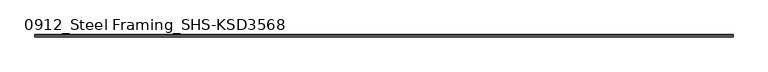
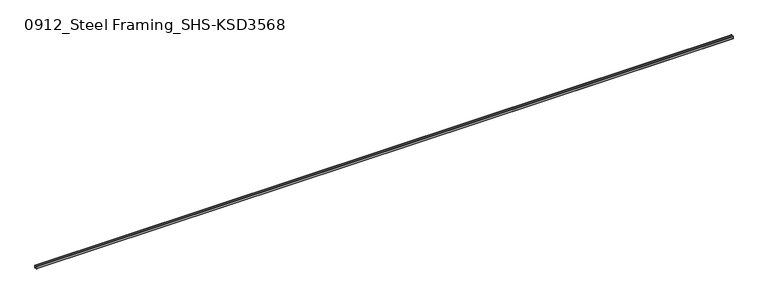
"""IFC4 building model written with IfcOpenShell, lengths in millimetres: beam geometry, 0912_Steel Framing_SHS-KSD3568 : H_SB_ASB_SHS-150x150x6."""

import ifcopenshell
import ifcopenshell.guid

model = None  # the IFC model being written
_history = None  # IfcOwnerHistory: only IFC2X3 demands one
_inside = {}  # id of a spatial element -> (the spatial element, [elements in it])
_under = {}  # id of a project, library or spatial element -> (it, [spatial elements below it])
_declared = {}  # id of a project -> (the project, [libraries it declares])
_typed = {}  # id of a type object -> (the type object, [elements of that type])
_made_of = {}  # id of a material, layer set ... -> (it, [elements and type objects made of it])


def new_model(schema):
    """Start an empty IFC model of exactly this schema.

    Asked for "IFC4X3", IfcOpenShell would pick the latest addendum, in which some entities
    have other attributes; the version numbers below select the first issue.
    IFC2X3 requires an IfcOwnerHistory on every rooted entity: one is made here for all.
    """
    global model, _history
    if schema == "IFC4X3":
        model = ifcopenshell.file(schema_version=(4, 3, 0, 0))
    else:
        model = ifcopenshell.file(schema=schema)
    _inside.clear()
    _under.clear()
    _declared.clear()
    _typed.clear()
    _made_of.clear()
    _history = None
    if model.schema == "IFC2X3":
        org = make("IfcOrganization", Name="unknown")
        user = make(
            "IfcPersonAndOrganization",
            ThePerson=make("IfcPerson", FamilyName="unknown"),
            TheOrganization=org,
        )
        app = make(
            "IfcApplication",
            ApplicationDeveloper=org,
            Version="unknown",
            ApplicationFullName="unknown",
            ApplicationIdentifier="unknown",
        )
        _history = make(
            "IfcOwnerHistory",
            OwningUser=user,
            OwningApplication=app,
            ChangeAction="ADDED",
            CreationDate=0,
        )
    return model


def make(cls, **values):
    """One entity of the class cls with the attributes given. An attribute that is None is left unset."""
    return model.create_entity(
        cls, **{name: value for name, value in values.items() if value is not None}
    )


def rooted(cls, **values):
    """An entity with a GlobalId (a new one), such as an element, a storey or a relation."""
    return make(cls, GlobalId=ifcopenshell.guid.new(), OwnerHistory=_history, **values)


def si_unit(unit_type, name, prefix=None):
    """IfcSIUnit, for example si_unit("LENGTHUNIT", "METRE", prefix="MILLI")."""
    return make("IfcSIUnit", UnitType=unit_type, Prefix=prefix, Name=name)


def assignment(units):
    """IfcUnitAssignment: the units of a project."""
    return None if units is None else make("IfcUnitAssignment", Units=units)


def point(xyz):
    """IfcCartesianPoint."""
    return None if xyz is None else make("IfcCartesianPoint", Coordinates=xyz)


def direction(xyz):
    """IfcDirection."""
    return None if xyz is None else make("IfcDirection", DirectionRatios=xyz)


def frame(location, z_axis=None, x_axis=None):
    """IfcAxis2Placement3D, a coordinate frame: its origin and axes. An axis left out is left unset."""
    return make(
        "IfcAxis2Placement3D",
        Location=point(location),
        Axis=direction(z_axis),
        RefDirection=direction(x_axis),
    )


def frame_2d(location, x_axis=None):
    """IfcAxis2Placement2D, a coordinate frame in the plane: its origin and x axis."""
    return make(
        "IfcAxis2Placement2D", Location=point(location), RefDirection=direction(x_axis)
    )


def origin():
    """The frame at (0, 0, 0) with its axes left unset."""
    return frame((0.0, 0.0, 0.0))


def place(relative_to, where):
    """IfcLocalPlacement: puts the frame where relative to a parent placement (None: the world)."""
    return make(
        "IfcLocalPlacement", PlacementRelTo=relative_to, RelativePlacement=where
    )


def context(
    kind, dimensions, precision=None, world=None, true_north=None, identifier=None
):
    """IfcGeometricRepresentationContext, for example the 3D "Model" context."""
    return make(
        "IfcGeometricRepresentationContext",
        ContextIdentifier=identifier,
        ContextType=kind,
        CoordinateSpaceDimension=dimensions,
        Precision=precision,
        WorldCoordinateSystem=world,
        TrueNorth=true_north,
    )


def project(units=None, contexts=None):
    """IfcProject with its units and contexts."""
    return rooted(
        "IfcProject",
        Name="project",
        RepresentationContexts=contexts,
        UnitsInContext=assignment(units),
    )


def spatial(cls, under=None, at=None, **own):
    """A site, building, storey or space (cls), placed at a placement, below another one or the project."""
    s = rooted(cls, ObjectPlacement=at, **own)
    if under is not None:
        _under.setdefault(under.id(), (under, []))[1].append(s)
    return s


def polyline(points):
    """IfcPolyline through the points."""
    return make("IfcPolyline", Points=[point(p) for p in points])


def circle_curve(where, radius):
    """IfcCircle in the frame where."""
    return make("IfcCircle", Position=where, Radius=radius)


def trimmed(basis, trim1, trim2, sense, master):
    """IfcTrimmedCurve: the piece of a basis curve between two trims."""
    return make(
        "IfcTrimmedCurve",
        BasisCurve=basis,
        Trim1=trim1,
        Trim2=trim2,
        SenseAgreement=sense,
        MasterRepresentation=master,
    )


def segment(curve, same_sense, transition):
    """IfcCompositeCurveSegment."""
    return make(
        "IfcCompositeCurveSegment",
        Transition=transition,
        SameSense=same_sense,
        ParentCurve=curve,
    )


def composite_curve(segments, self_intersect=None):
    """IfcCompositeCurve: segments joined end to end."""
    return make("IfcCompositeCurve", Segments=segments, SelfIntersect=self_intersect)


def outline(outer, holes=None, kind="AREA"):
    """IfcArbitraryClosedProfileDef: a profile drawn as a closed curve; with holes, ...WithVoids."""
    if holes is None:
        return make("IfcArbitraryClosedProfileDef", ProfileType=kind, OuterCurve=outer)
    return make(
        "IfcArbitraryProfileDefWithVoids",
        ProfileType=kind,
        OuterCurve=outer,
        InnerCurves=holes,
    )


def extrude(swept, where, along, depth):
    """IfcExtrudedAreaSolid: the profile swept, set in the frame where, extruded along a direction by depth."""
    return make(
        "IfcExtrudedAreaSolid",
        SweptArea=swept,
        Position=where,
        ExtrudedDirection=direction(along),
        Depth=depth,
    )


def shape(context_of_items, identifier, shape_type, items):
    """IfcShapeRepresentation: the items that make up one representation, for example the "Body"."""
    return make(
        "IfcShapeRepresentation",
        ContextOfItems=context_of_items,
        RepresentationIdentifier=identifier,
        RepresentationType=shape_type,
        Items=items,
    )


def source(mapping_origin, context_of_items, identifier, shape_type, items):
    """IfcRepresentationMap: a shape defined once, which mapped items show again and again."""
    return make(
        "IfcRepresentationMap",
        MappingOrigin=mapping_origin,
        MappedRepresentation=shape(context_of_items, identifier, shape_type, items),
    )


def transform(
    local_origin,
    x_axis=None,
    y_axis=None,
    z_axis=None,
    scale=None,
    scale2=None,
    scale3=None,
    uniform=True,
):
    """IfcCartesianTransformationOperator3D, or its non-uniform kind. x_axis, y_axis, z_axis: its Axis1, 2, 3."""
    if uniform:
        return make(
            "IfcCartesianTransformationOperator3D",
            Axis1=direction(x_axis),
            Axis2=direction(y_axis),
            LocalOrigin=point(local_origin),
            Scale=scale,
            Axis3=direction(z_axis),
        )
    return make(
        "IfcCartesianTransformationOperator3DnonUniform",
        Axis1=direction(x_axis),
        Axis2=direction(y_axis),
        LocalOrigin=point(local_origin),
        Scale=scale,
        Axis3=direction(z_axis),
        Scale2=scale2,
        Scale3=scale3,
    )


def mapped(mapping_source, mapping_target):
    """IfcMappedItem: shows the shape of a source again, moved by a transform."""
    return make(
        "IfcMappedItem", MappingSource=mapping_source, MappingTarget=mapping_target
    )


def made_of(thing, what):
    """Note that an element or type object is made of a material, layer set ...; save() writes the relation."""
    if what is not None:
        _made_of.setdefault(what.id(), (what, []))[1].append(thing)
    return thing


def element(
    cls,
    number,
    at=None,
    inside=None,
    cuts=None,
    type_object=None,
    material=None,
    context=None,
    identifier="Body",
    shape_type=None,
    held_by="IfcProductDefinitionShape",
    body=None,
    shapes=None,
    **own,
):
    """One element of the class cls, such as IfcWall. Its Tag is "e" and its number.

    at: its placement. inside: the storey or other place that contains it. cuts: it is an
    opening in that element (IfcRelVoidsElement). A single representation is given by context,
    identifier, shape_type and body (its items); several are given by shapes. held_by: the class
    of the entity that holds the representations. save() writes the other relations.
    """
    e = rooted(cls, Tag="e%d" % number, ObjectPlacement=at, **own)
    if body is not None:
        shapes = [shape(context, identifier, shape_type, body)]
    if shapes is not None:
        e.Representation = make(held_by, Representations=shapes)
    if inside is not None:
        _inside.setdefault(inside.id(), (inside, []))[1].append(e)
    if cuts is not None:
        rooted(
            "IfcRelVoidsElement", RelatingBuildingElement=cuts, RelatedOpeningElement=e
        )
    if type_object is not None:
        _typed.setdefault(type_object.id(), (type_object, []))[1].append(e)
    return made_of(e, material)


def aggregate(whole, parts):
    """IfcRelAggregates: a whole, such as a stair, and the parts it consists of."""
    return rooted("IfcRelAggregates", RelatingObject=whole, RelatedObjects=parts)


def save(model, path):
    """Write the relations noted so far, then the file.

    IfcRelAggregates (storeys below a building ...), IfcRelContainedInSpatialStructure (elements
    in a storey), IfcRelDefinesByType, IfcRelAssociatesMaterial and IfcRelDeclares: one each for
    every whole, place, type object, material and project.
    """
    for whole, parts in _under.values():
        aggregate(whole, parts)
    for where, things in _inside.values():
        rooted(
            "IfcRelContainedInSpatialStructure",
            RelatedElements=things,
            RelatingStructure=where,
        )
    for kind, things in _typed.values():
        rooted("IfcRelDefinesByType", RelatedObjects=things, RelatingType=kind)
    for what, things in _made_of.values():
        rooted("IfcRelAssociatesMaterial", RelatedObjects=things, RelatingMaterial=what)
    for by, libraries in _declared.values():
        rooted("IfcRelDeclares", RelatingContext=by, RelatedDefinitions=libraries)
    model.write(path)


def beam_0912_steel_framing_shs_ksd3568_92ad3d46(model_context):
    return source(origin(), model_context, "Body", "SweptSolid", [
        extrude(outline(composite_curve([segment(polyline([(75.0, 63.0), (75.0, -63.0)]), True, "CONTINUOUS"), segment(trimmed(circle_curve(frame_2d((63.0, -63.0)), 12.0), [point((75.0, -63.0))], [point((63.0, -75.0))], False, "CARTESIAN"), True, "CONTINUOUS"), segment(polyline([(63.0, -75.0), (-63.0, -75.0)]), True, "CONTINUOUS"), segment(trimmed(circle_curve(frame_2d((-63.0, -63.0)), 12.0), [point((-63.0, -75.0))], [point((-75.0, -63.0))], False, "CARTESIAN"), True, "CONTINUOUS"), segment(polyline([(-75.0, -63.0), (-75.0, 63.0)]), True, "CONTINUOUS"), segment(trimmed(circle_curve(frame_2d((-63.0, 63.0)), 12.0), [point((-75.0, 63.0))], [point((-63.0, 75.0))], False, "CARTESIAN"), True, "CONTINUOUS"), segment(polyline([(-63.0, 75.0), (63.0, 75.0)]), True, "CONTINUOUS"), segment(trimmed(circle_curve(frame_2d((63.0, 63.0)), 12.0), [point((63.0, 75.0))], [point((75.0, 63.0))], False, "CARTESIAN"), True, "CONTINUOUS")], self_intersect=False), holes=[composite_curve([segment(trimmed(circle_curve(frame_2d((-63.0, 63.0)), 6.0), [point((-63.0, 69.0))], [point((-69.0, 63.0))], True, "CARTESIAN"), True, "CONTINUOUS"), segment(polyline([(-69.0, 63.0), (-69.0, -63.0)]), True, "CONTINUOUS"), segment(trimmed(circle_curve(frame_2d((-63.0, -63.0)), 6.0), [point((-69.0, -63.0))], [point((-63.0, -69.0))], True, "CARTESIAN"), True, "CONTINUOUS"), segment(polyline([(-63.0, -69.0), (63.0, -69.0)]), True, "CONTINUOUS"), segment(trimmed(circle_curve(frame_2d((63.0, -63.0)), 6.0), [point((63.0, -69.0))], [point((69.0, -63.0))], True, "CARTESIAN"), True, "CONTINUOUS"), segment(polyline([(69.0, -63.0), (69.0, 63.0)]), True, "CONTINUOUS"), segment(trimmed(circle_curve(frame_2d((63.0, 63.0)), 6.0), [point((69.0, 63.0))], [point((63.0, 69.0))], True, "CARTESIAN"), True, "CONTINUOUS"), segment(polyline([(63.0, 69.0), (-63.0, 69.0)]), True, "CONTINUOUS")], self_intersect=False)]), frame((-20440.0, 0.0, 0.0), z_axis=(1.0, 0.0, 0.0), x_axis=(0.0, 1.0, 0.0)), (0.0, 0.0, 1.0), 40880.0),
    ])


if __name__ == "__main__":
    model = new_model("IFC4")
    model_context = context("Model", 3, world=origin())
    ifc_project = project(units=[si_unit("LENGTHUNIT", "METRE", prefix="MILLI")], contexts=[model_context])
    site = spatial("IfcSite", under=ifc_project)
    building = spatial("IfcBuilding", under=site)
    placement = place(None, origin())
    beam_0912_steel_framing_shs_ksd3568_shape = beam_0912_steel_framing_shs_ksd3568_92ad3d46(model_context)
    element("IfcBeam", 1, ObjectType="0912_Steel Framing_SHS-KSD3568 : H_SB_ASB_SHS-150x150x6", at=placement, inside=building, context=model_context, shape_type="MappedRepresentation", body=[
        mapped(beam_0912_steel_framing_shs_ksd3568_shape, transform((0.0, 0.0, 0.0), x_axis=(1.0, 0.0, 0.0), y_axis=(0.0, 1.0, 0.0), z_axis=(0.0, 0.0, 1.0))),
    ])
    save(model, "model.ifc")

# Revit data of these elements
# Type "0912_Steel Framing_SHS-KSD3568 : H_SB_ASB_SHS-150x150x6"
#   H_WM Code_1 = "S01AA002-00001 | Main Steel Structure Fabrication Work | Shelter/Building | Medium Steel - Standard (90KG/M>Weight≥30KG/M) | Material: (   )"
#   H_WM Code_2 = "S03AA028-00001 | Main Steel Structure Erection Work | Shelter/Building | Medium Steel (90KG/M>Weight≥30KG/M) | Material: (   )"
#   H_WM Code_3 = "S01AA010-00001 | Main Steel Structure Fabrication Work | Shelter/Building | Steel Painting/Coating | for Non-Fireproofed Steel Surface, Surface Preparation, Primer, Second & Final Coat | Material: (   )"
#   H_Q'ty Cal Type Tag = "SB-Q2"
#   Perimeter = 0.60 m²/m
#   Nominal Weight = 26.40 kgf/m
#   Length [instance default] = 1.0000 m
#   b = 0.1500 m
#   h = 0.1500 m
#   tr = 0.0120 m
#   t = 0.0060 m
#   A = 28.36 m²
#   Structural Material [instance default] = Steel, 45-345
# Element 1 (IfcBeam, "0912_Steel Framing_SHS-KSD3568 : H_SB_ASB_SHS-150x150x6")
#   Structural Material = none
# Materials
#   "Steel, 45-345": class "Metal", colour RGB 189 187 185, transparency 0, Description = "Steel 345 MPa", Cost = 0
